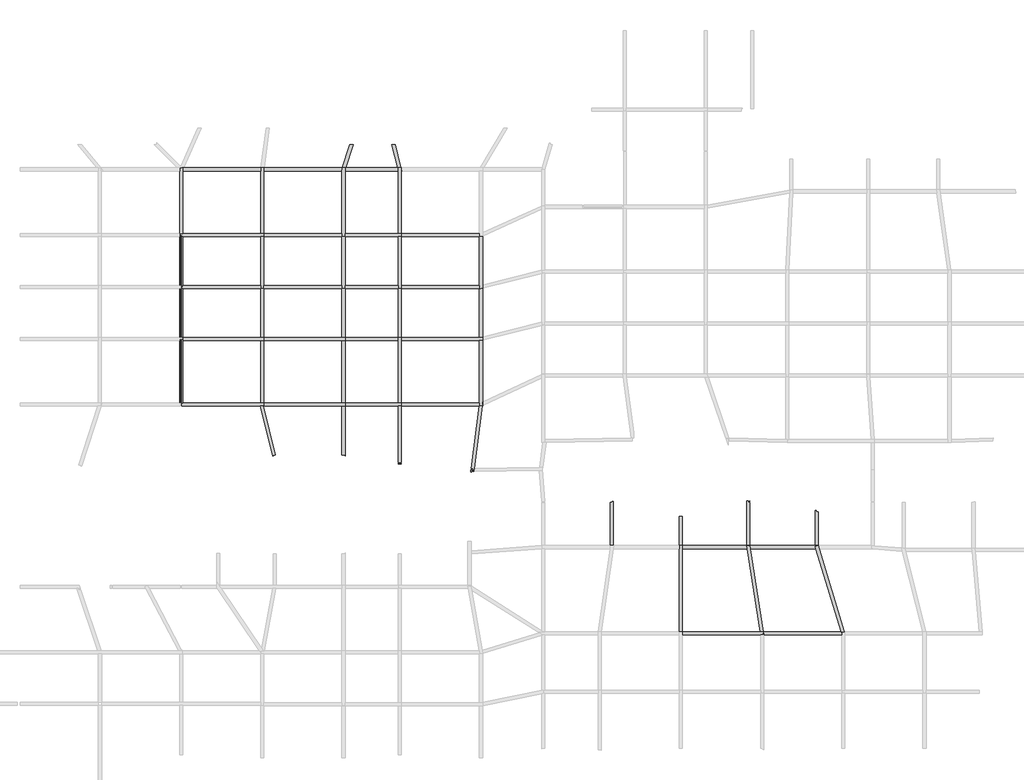
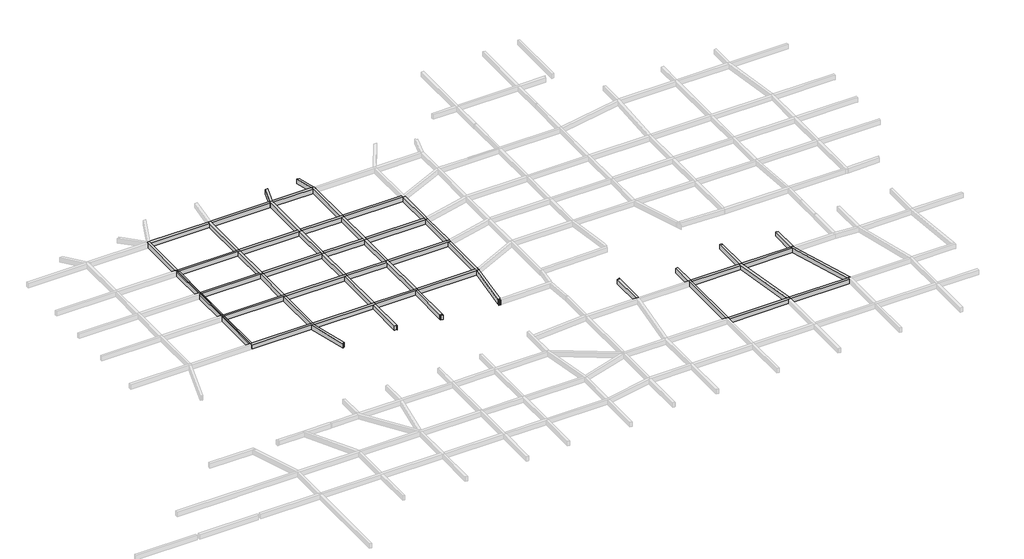
# One storey, part 11 of 15: 55 beams.
"""IFC4 building model written with IfcOpenShell, lengths in millimetres."""

from ifc_helpers import new_model, si_unit, frame, origin, place, context, project, spatial, polyline, outline, extrude, faceted_brep, element, save

model = new_model("IFC4")

# Units and contexts
model_context = context("Model", 3, world=origin())
ifc_project = project(units=[si_unit("LENGTHUNIT", "METRE", prefix="MILLI")], contexts=[model_context])

# Site, building, storey
site = spatial("IfcSite", under=ifc_project)
building = spatial("IfcBuilding", under=site)
storey = spatial("IfcBuildingStorey", under=building, Name="层高", Elevation=3300.0)

# Beams
placement = place(None, origin())
element("IfcBeam", 1, ObjectType="混凝土 - 矩形梁 : KL_beam", at=placement, inside=storey, context=model_context, shape_type="Brep", body=[
    faceted_brep([(192640.3009401, 110342.1448334, 3300.0), (192550.3215993, 110342.1448334, 3300.0), (192550.3215993, 110192.1448334, 3300.0), (192550.3215993, 104192.1448334, 3300.0), (192640.3009401, 104192.1448334, 3300.0), (192550.3215993, 104192.1448334, 2700.0), (192550.3215993, 110342.1448334, 2700.0), (192550.3215993, 110192.1448334, 2700.0), (192640.3009401, 104192.1448334, 2700.0), (192640.3009401, 110342.1448334, 2700.0)], [[[0, 1, 2, 3, 4]], [[5, 3, 2, 1, 6, 7]], [[3, 5, 8, 4]], [[0, 4, 8, 9]], [[8, 5, 7, 6, 9]], [[6, 1, 0, 9]]]),
    faceted_brep([(192850.3215993, 110342.1448334, 2700.0), (192850.3215993, 110342.1448334, 3300.0), (192850.3215993, 110192.1448334, 3300.0), (192850.3215993, 104192.1448334, 3300.0), (192850.3215993, 104192.1448334, 2700.0), (192850.3215993, 110192.1448334, 2700.0), (192760.3009401, 110342.1448334, 2700.0), (192760.3009401, 104192.1448334, 2700.0), (192760.3009401, 110342.1448334, 3300.0), (192760.3009401, 104192.1448334, 3300.0)], [[[0, 1, 2, 3, 4, 5]], [[6, 0, 5, 4, 7]], [[1, 0, 6, 8]], [[8, 6, 7, 9]], [[1, 8, 9, 3, 2]], [[4, 3, 9, 7]]]),
])
element("IfcBeam", 2, ObjectType="混凝土 - 矩形梁 : KL_beam", at=placement, inside=storey, context=model_context, shape_type="Brep", body=[
    faceted_brep([(192850.3009401, 110492.1448334, 3300.0), (192850.3112697, 110342.1448326, 3300.0), (192850.3215993, 110192.1448334, 3300.0), (200350.3215993, 110192.1448334, 3300.0), (200650.3215993, 110192.1448334, 3300.0), (200650.3215993, 110492.1448334, 3300.0), (200350.3009401, 110492.1448334, 3300.0), (192850.3215993, 110192.1448334, 2700.0), (200350.3215993, 110192.1448334, 2700.0), (200650.3215993, 110192.1448334, 2700.0), (192850.3112697, 110342.1448326, 2700.0), (192850.3009401, 110492.1448334, 2700.0), (200350.3009401, 110492.1448334, 2700.0), (200650.3215993, 110492.1448334, 2700.0)], [[[0, 1, 2, 3, 4, 5, 6]], [[2, 7, 8, 9, 4, 3]], [[7, 10, 11, 12, 13, 9, 8]], [[5, 13, 12, 11, 0, 6]], [[0, 11, 10, 7, 2, 1]], [[5, 4, 9, 13]]]),
])
element("IfcBeam", 3, ObjectType="混凝土 - 矩形梁 : KL_beam", at=placement, inside=storey, context=model_context, shape_type="Brep", body=[
    faceted_brep([(200650.3215993, 103892.1448334, 3300.0), (200650.3215993, 104192.1448334, 3300.0), (200350.3215993, 104192.1448334, 3300.0), (192850.3215993, 104192.1448334, 3300.0), (192760.3009401, 104192.1448334, 3300.0), (192760.3009401, 103892.1448334, 3300.0), (200283.1287554, 103892.1448334, 3300.0), (200592.3128442, 103892.1448334, 3300.0), (200650.3215993, 103892.1448334, 2700.0), (192760.3009401, 103892.1448334, 2700.0), (200283.1287554, 103892.1448334, 2700.0), (200592.3128442, 103892.1448334, 2700.0), (200650.3215993, 104192.1448334, 2700.0), (192760.3009401, 104192.1448334, 2700.0), (192850.3215993, 104192.1448334, 2700.0), (200350.3215993, 104192.1448334, 2700.0)], [[[0, 1, 2, 3, 4, 5, 6, 7]], [[8, 0, 7, 6, 5, 9, 10, 11]], [[12, 8, 11, 10, 9, 13, 14, 15]], [[1, 12, 15, 14, 13, 4, 3, 2]], [[1, 0, 8, 12]], [[5, 4, 13, 9]]]),
])
element("IfcBeam", 4, ObjectType="混凝土 - 矩形梁 : KL_beam", at=placement, inside=storey, context=model_context, shape_type="SweptSolid", body=[
    extrude(outline(polyline([(200350.3215993, 110192.1448334), (200650.3215993, 110192.1448334), (200650.3215993, 104192.1448334), (200350.3215993, 104192.1448334), (200350.3215993, 110192.1448334)])), frame((0.0, 0.0, 2700.0), z_axis=(0.0, 0.0, 1.0), x_axis=(1.0, 0.0, 0.0)), (0.0, 0.0, 1.0), 600.0),
])
element("IfcBeam", 5, ObjectType="混凝土 - 矩形梁 : KL_beam", at=placement, inside=storey, context=model_context, shape_type="Brep", body=[
    faceted_brep([(208450.3009398, 103892.1448334, 3300.0), (208450.3009398, 104192.1448334, 3300.0), (208150.3009398, 104192.1448334, 3300.0), (200650.3215993, 104192.1448334, 3300.0), (200650.3215993, 103892.1448334, 3300.0), (208150.3009398, 103892.1448334, 3300.0), (208450.3009398, 103892.1448334, 2700.0), (200650.3215993, 103892.1448334, 2700.0), (208150.3009398, 103892.1448334, 2700.0), (208450.3009398, 104192.1448334, 2700.0), (200650.3215993, 104192.1448334, 2700.0), (208150.3009398, 104192.1448334, 2700.0)], [[[0, 1, 2, 3, 4, 5]], [[6, 0, 5, 4, 7, 8]], [[9, 6, 8, 7, 10, 11]], [[1, 9, 11, 10, 3, 2]], [[4, 3, 10, 7]], [[1, 0, 6, 9]]]),
])
element("IfcBeam", 6, ObjectType="混凝土 - 矩形梁 : KL_beam", at=placement, inside=storey, context=model_context, shape_type="Brep", body=[
    faceted_brep([(208450.3009398, 110192.1448334, 3300.0), (208450.3009398, 110492.1448334, 3300.0), (208150.3009398, 110492.1448334, 3300.0), (200650.3215993, 110492.1448334, 3300.0), (200650.3215993, 110192.1448334, 3300.0), (208150.3009398, 110192.1448334, 3300.0), (208450.3009398, 110192.1448334, 2700.0), (200650.3215993, 110192.1448334, 2700.0), (208150.3009398, 110192.1448334, 2700.0), (208450.3009398, 110492.1448334, 2700.0), (200650.3215993, 110492.1448334, 2700.0), (208150.3009398, 110492.1448334, 2700.0)], [[[0, 1, 2, 3, 4, 5]], [[6, 0, 5, 4, 7, 8]], [[9, 6, 8, 7, 10, 11]], [[1, 9, 11, 10, 3, 2]], [[4, 3, 10, 7]], [[1, 0, 6, 9]]]),
])
element("IfcBeam", 7, ObjectType="混凝土 - 矩形梁 : KL_beam", at=placement, inside=storey, context=model_context, shape_type="SweptSolid", body=[
    extrude(outline(polyline([(208450.3009398, 104192.1448334), (208150.3009398, 104192.1448334), (208150.3009398, 110192.1448334), (208450.3009398, 110192.1448334), (208450.3009398, 104192.1448334)])), frame((0.0, 0.0, 2700.0), z_axis=(0.0, 0.0, 1.0), x_axis=(1.0, 0.0, 0.0)), (0.0, 0.0, 1.0), 600.0),
])
element("IfcBeam", 8, ObjectType="混凝土 - 矩形梁 : KL_beam", at=placement, inside=storey, context=model_context, shape_type="Brep", body=[
    faceted_brep([(213850.3009384, 103892.1448334, 3300.0), (213850.3009384, 104192.1448334, 3300.0), (213550.3009384, 104192.1448334, 3300.0), (208450.3009398, 104192.1448334, 3300.0), (208450.3009398, 103892.1448334, 3300.0), (213550.3009384, 103892.1448334, 3300.0), (213850.3009384, 103892.1448334, 2700.0), (208450.3009398, 103892.1448334, 2700.0), (213550.3009384, 103892.1448334, 2700.0), (213850.3009384, 104192.1448334, 2700.0), (208450.3009398, 104192.1448334, 2700.0), (213550.3009384, 104192.1448334, 2700.0)], [[[0, 1, 2, 3, 4, 5]], [[6, 0, 5, 4, 7, 8]], [[9, 6, 8, 7, 10, 11]], [[1, 9, 11, 10, 3, 2]], [[4, 3, 10, 7]], [[1, 0, 6, 9]]]),
])
element("IfcBeam", 9, ObjectType="混凝土 - 矩形梁 : KL_beam", at=placement, inside=storey, context=model_context, shape_type="Brep", body=[
    faceted_brep([(213850.3009384, 110492.1448334, 3300.0), (213550.3009384, 110492.1448334, 3300.0), (213550.3009384, 110192.1448334, 3300.0), (213550.3009384, 104192.1448334, 3300.0), (213850.3009384, 104192.1448334, 3300.0), (213850.3009384, 110192.1448334, 3300.0), (213850.3009384, 110492.1448334, 2700.0), (213850.3009384, 104192.1448334, 2700.0), (213850.3009384, 110192.1448334, 2700.0), (213550.3009384, 110492.1448334, 2700.0), (213550.3009384, 104192.1448334, 2700.0), (213550.3009384, 110192.1448334, 2700.0)], [[[0, 1, 2, 3, 4, 5]], [[6, 0, 5, 4, 7, 8]], [[9, 6, 8, 7, 10, 11]], [[1, 9, 11, 10, 3, 2]], [[4, 3, 10, 7]], [[1, 0, 6, 9]]]),
])
element("IfcBeam", 10, ObjectType="混凝土 - 矩形梁 : KL_beam", at=placement, inside=storey, context=model_context, shape_type="SweptSolid", body=[
    extrude(outline(polyline([(208450.3009398, 110192.1448334), (208450.3009398, 110492.1448334), (213550.3009384, 110492.1448334), (213550.3009384, 110192.1448334), (208450.3009398, 110192.1448334)])), frame((0.0, 0.0, 2700.0), z_axis=(0.0, 0.0, 1.0), x_axis=(1.0, 0.0, 0.0)), (0.0, 0.0, 1.0), 600.0),
])
element("IfcBeam", 11, ObjectType="混凝土 - 矩形梁 : KL_beam", at=placement, inside=storey, context=model_context, shape_type="SweptSolid", body=[
    extrude(outline(polyline([(213850.3009384, 98342.0955388), (213550.3009384, 98342.0955388), (213550.3009384, 98382.0955388), (213850.3009384, 98382.0955388), (213850.3009384, 98342.0955388)])), frame((0.0, 0.0, 2700.0), z_axis=(0.0, 0.0, 1.0), x_axis=(1.0, 0.0, 0.0)), (0.0, 0.0, 1.0), 600.0),
    extrude(outline(polyline([(213550.3009384, 103892.1448334), (213850.3009384, 103892.1448334), (213850.3009384, 98502.0955388), (213550.3009384, 98502.0955388), (213550.3009384, 103892.1448334)])), frame((0.0, 0.0, 2700.0), z_axis=(0.0, 0.0, 1.0), x_axis=(1.0, 0.0, 0.0)), (0.0, 0.0, 1.0), 600.0),
])
element("IfcBeam", 12, ObjectType="混凝土 - 矩形梁 : KL_beam", at=placement, inside=storey, context=model_context, shape_type="Brep", body=[
    faceted_brep([(208450.3009398, 103892.1448334, 3300.0), (208150.3009398, 103892.1448334, 3300.0), (208150.3009398, 99202.0955388, 3300.0), (208329.2467743, 99202.0955388, 3300.0), (208449.2467743, 99202.0955388, 3300.0), (208449.2467743, 99082.0955388, 3300.0), (208450.3009398, 99082.0955388, 3300.0), (208150.3009398, 103892.1448334, 2700.0), (208150.3009398, 99202.0955388, 2700.0), (208450.3009398, 103892.1448334, 2700.0), (208450.3009398, 99082.0955388, 2700.0), (208449.2467743, 99082.0955388, 2700.0), (208449.2467743, 99202.0955388, 2700.0)], [[[0, 1, 2, 3, 4, 5, 6]], [[1, 7, 8, 2]], [[7, 9, 10, 11, 12, 8]], [[9, 0, 6, 10]], [[1, 0, 9, 7]], [[10, 6, 5, 11]], [[2, 8, 12, 4, 3]], [[4, 12, 11, 5]]]),
])
element("IfcBeam", 13, ObjectType="混凝土 - 矩形梁 : KL_beam", at=placement, inside=storey, context=model_context, shape_type="SweptSolid", body=[
    extrude(outline(polyline([(200283.1287554, 103892.1448334), (200592.3128442, 103892.1448334), (201761.673468, 99202.0955388), (201562.0411038, 99202.0955388), (201562.0411038, 99082.0955388), (201482.4087396, 99082.0955388), (200283.1287554, 103892.1448334)])), frame((0.0, 0.0, 2700.0), z_axis=(0.0, 0.0, 1.0), x_axis=(1.0, 0.0, 0.0)), (0.0, 0.0, 1.0), 600.0),
])
element("IfcBeam", 14, ObjectType="混凝土 - 矩形梁 : KL_beam", at=placement, inside=storey, context=model_context, shape_type="Brep", body=[
    faceted_brep([(200650.3009401, 120192.1448334, 3300.0), (200650.3009401, 120492.1448334, 3300.0), (200350.3009384, 120492.1448334, 3300.0), (192850.3052169, 120492.1448334, 3300.0), (192550.3009401, 120492.1448334, 3300.0), (192550.3009401, 120192.1448334, 3300.0), (192640.3009401, 120192.1448334, 3300.0), (192640.3009401, 120342.1448334, 3300.0), (192760.3009401, 120342.1448334, 3300.0), (192760.3009401, 120192.1448334, 3300.0), (192850.3009401, 120192.1448334, 3300.0), (200350.3009401, 120192.1448334, 3300.0), (200650.3009401, 120192.1448334, 2700.0), (192760.3009401, 120192.1448334, 2700.0), (192850.3009401, 120192.1448334, 2700.0), (200350.3009401, 120192.1448334, 2700.0), (200650.3009401, 120492.1448334, 2700.0), (192760.3009401, 120342.1448334, 2700.0), (192640.3009401, 120342.1448334, 2700.0), (192640.3009401, 120192.1448334, 2700.0), (192550.3009401, 120192.1448334, 2700.0), (192550.3009401, 120492.1448334, 2700.0), (192850.3052169, 120492.1448334, 2700.0), (200350.3009384, 120492.1448334, 2700.0)], [[[0, 1, 2, 3, 4, 5, 6, 7, 8, 9, 10, 11]], [[12, 0, 11, 10, 9, 13, 14, 15]], [[16, 12, 15, 14, 13, 17, 18, 19, 20, 21, 22, 23]], [[1, 16, 23, 22, 21, 4, 3, 2]], [[1, 0, 12, 16]], [[5, 4, 21, 20]], [[18, 7, 6, 19]], [[8, 17, 13, 9]], [[7, 18, 17, 8]], [[5, 20, 19, 6]]]),
])
element("IfcBeam", 15, ObjectType="混凝土 - 矩形梁 : KL_beam", at=placement, inside=storey, context=model_context, shape_type="Brep", body=[
    faceted_brep([(200350.3009401, 115192.1448334, 3300.0), (200650.3009401, 115192.1448334, 3300.0), (200650.3009401, 115492.1448334, 3300.0), (200650.3009401, 120192.1448334, 3300.0), (200350.3009401, 120192.1448334, 3300.0), (200350.3009401, 115492.1448334, 3300.0), (200350.3009401, 115192.1448334, 2700.0), (200350.3009401, 120192.1448334, 2700.0), (200350.3009401, 115492.1448334, 2700.0), (200650.3009401, 115192.1448334, 2700.0), (200650.3009401, 120192.1448334, 2700.0), (200650.3009401, 115492.1448334, 2700.0)], [[[0, 1, 2, 3, 4, 5]], [[6, 0, 5, 4, 7, 8]], [[9, 6, 8, 7, 10, 11]], [[1, 9, 11, 10, 3, 2]], [[4, 3, 10, 7]], [[1, 0, 6, 9]]]),
])
element("IfcBeam", 16, ObjectType="混凝土 - 矩形梁 : KL_beam", at=placement, inside=storey, context=model_context, shape_type="Brep", body=[
    faceted_brep([(200650.3009384, 126792.1448334, 3300.0), (200368.9005343, 126792.1448334, 3300.0), (200350.3009384, 126792.1448334, 3300.0), (200350.3009384, 126492.1448334, 3300.0), (200350.3009384, 120492.1448334, 3300.0), (200650.3009384, 120492.1448334, 3300.0), (200650.3009384, 126492.1448334, 3300.0), (200350.3009384, 126792.1448334, 2700.0), (200350.3009384, 126492.1448334, 2700.0), (200350.3009384, 120492.1448334, 2700.0), (200368.9005343, 126792.1448334, 2700.0), (200650.3009384, 126792.1448334, 2700.0), (200650.3009384, 126492.1448334, 2700.0), (200650.3009384, 120492.1448334, 2700.0)], [[[0, 1, 2, 3, 4, 5, 6]], [[2, 7, 8, 9, 4, 3]], [[7, 10, 11, 12, 13, 9, 8]], [[11, 0, 6, 5, 13, 12]], [[5, 4, 9, 13]], [[2, 1, 0, 11, 10, 7]]]),
])
element("IfcBeam", 17, ObjectType="混凝土 - 矩形梁 : KL_beam", at=placement, inside=storey, context=model_context, shape_type="Brep", body=[
    faceted_brep([(192850.3052169, 126792.1448334, 3300.0), (192762.4372513, 126792.1448334, 3300.0), (192550.3052169, 126792.1448334, 3300.0), (192550.3052169, 126492.1448334, 3300.0), (192550.3052169, 120492.1448334, 3300.0), (192850.3052169, 120492.1448334, 3300.0), (192850.3052169, 126492.1448334, 3300.0), (192550.3052169, 126792.1448334, 2700.0), (192550.3052169, 126492.1448334, 2700.0), (192550.3052169, 120492.1448334, 2700.0), (192762.4372513, 126792.1448334, 2700.0), (192850.3052169, 126792.1448334, 2700.0), (192850.3052169, 126492.1448334, 2700.0), (192850.3052169, 120492.1448334, 2700.0)], [[[0, 1, 2, 3, 4, 5, 6]], [[2, 7, 8, 9, 4, 3]], [[7, 10, 11, 12, 13, 9, 8]], [[11, 0, 6, 5, 13, 12]], [[5, 4, 9, 13]], [[2, 1, 0, 11, 10, 7]]]),
])
element("IfcBeam", 18, ObjectType="混凝土 - 矩形梁 : KL_beam", at=placement, inside=storey, context=model_context, shape_type="Brep", body=[
    faceted_brep([(200350.3009384, 126492.1448334, 3300.0), (200350.3009384, 126792.1448334, 3300.0), (192931.5266601, 126792.1448334, 3300.0), (192850.3052169, 126792.1448334, 3300.0), (192850.3052169, 126492.1448334, 3300.0), (200350.3009384, 126492.1448334, 2700.0), (192850.3052169, 126492.1448334, 2700.0), (200350.3009384, 126792.1448334, 2700.0), (192850.3052169, 126792.1448334, 2700.0), (192931.5266601, 126792.1448334, 2700.0)], [[[0, 1, 2, 3, 4]], [[5, 0, 4, 6]], [[7, 5, 6, 8, 9]], [[1, 7, 9, 8, 3, 2]], [[1, 0, 5, 7]], [[4, 3, 8, 6]]]),
])
element("IfcBeam", 19, ObjectType="混凝土 - 矩形梁 : KL_beam", at=placement, inside=storey, context=model_context, shape_type="Brep", body=[
    faceted_brep([(208150.3009398, 120192.1448334, 3300.0), (208450.3009398, 120192.1448334, 3300.0), (208450.3009398, 120492.1448334, 3300.0), (208450.3009398, 126492.1448334, 3300.0), (208450.3009398, 126792.1448334, 3300.0), (208191.3195606, 126792.1448334, 3300.0), (208150.3009398, 126792.1448334, 3300.0), (208150.3009398, 126665.9024994, 3300.0), (208150.3009398, 126492.1448334, 3300.0), (208150.3009398, 120492.1448334, 3300.0), (208150.3009398, 120192.1448334, 2700.0), (208150.3009398, 126792.1448334, 2700.0), (208150.3009398, 126665.9024994, 2700.0), (208150.3009398, 126492.1448334, 2700.0), (208150.3009398, 120492.1448334, 2700.0), (208450.3009398, 120192.1448334, 2700.0), (208191.3195606, 126792.1448334, 2700.0), (208450.3009398, 126792.1448334, 2700.0), (208450.3009398, 126492.1448334, 2700.0), (208450.3009398, 120492.1448334, 2700.0)], [[[0, 1, 2, 3, 4, 5, 6, 7, 8, 9]], [[10, 0, 9, 8, 7, 6, 11, 12, 13, 14]], [[15, 10, 14, 13, 12, 11, 16, 17, 18, 19]], [[1, 15, 19, 18, 17, 4, 3, 2]], [[1, 0, 10, 15]], [[6, 5, 4, 17, 16, 11]]]),
])
element("IfcBeam", 20, ObjectType="混凝土 - 矩形梁 : KL_beam", at=placement, inside=storey, context=model_context, shape_type="Brep", body=[
    faceted_brep([(213850.3009384, 120192.1448334, 3300.0), (213850.3009384, 120492.1448334, 3300.0), (213550.3009384, 120492.1448334, 3300.0), (208450.3009398, 120492.1448334, 3300.0), (208450.3009398, 120192.1448334, 3300.0), (213550.3009384, 120192.1448334, 3300.0), (213850.3009384, 120192.1448334, 2700.0), (208450.3009398, 120192.1448334, 2700.0), (213550.3009384, 120192.1448334, 2700.0), (213850.3009384, 120492.1448334, 2700.0), (208450.3009398, 120492.1448334, 2700.0), (213550.3009384, 120492.1448334, 2700.0)], [[[0, 1, 2, 3, 4, 5]], [[6, 0, 5, 4, 7, 8]], [[9, 6, 8, 7, 10, 11]], [[1, 9, 11, 10, 3, 2]], [[4, 3, 10, 7]], [[1, 0, 6, 9]]]),
])
element("IfcBeam", 21, ObjectType="混凝土 - 矩形梁 : KL_beam", at=placement, inside=storey, context=model_context, shape_type="Brep", body=[
    faceted_brep([(213850.3009384, 126792.1448334, 3300.0), (213817.4937825, 126792.1448334, 3300.0), (213550.3009384, 126792.1448334, 3300.0), (213550.3009384, 126492.1448334, 3300.0), (213550.3009384, 120492.1448334, 3300.0), (213850.3009384, 120492.1448334, 3300.0), (213850.3009384, 126492.1448336, 3300.0), (213850.3009384, 126660.5625177, 3300.0), (213550.3009384, 126792.1448334, 2700.0), (213550.3009384, 126492.1448334, 2700.0), (213550.3009384, 120492.1448334, 2700.0), (213817.4937825, 126792.1448334, 2700.0), (213850.3009384, 126792.1448334, 2700.0), (213850.3009384, 126660.5625177, 2700.0), (213850.3009384, 126492.1448336, 2700.0), (213850.3009384, 120492.1448334, 2700.0)], [[[0, 1, 2, 3, 4, 5, 6, 7]], [[2, 8, 9, 10, 4, 3]], [[8, 11, 12, 13, 14, 15, 10, 9]], [[12, 0, 7, 6, 5, 15, 14, 13]], [[5, 4, 10, 15]], [[2, 1, 0, 12, 11, 8]]]),
])
element("IfcBeam", 22, ObjectType="混凝土 - 矩形梁 : KL_beam", at=placement, inside=storey, context=model_context, shape_type="Brep", body=[
    faceted_brep([(208450.3009398, 126792.1448334, 3300.0), (208450.3009398, 126492.1448334, 3300.0), (213550.3009384, 126492.1448334, 3300.0), (213550.3009384, 126792.1448334, 3300.0), (213508.3096937, 126792.1448334, 3300.0), (208506.7582279, 126792.1448334, 3300.0), (208450.3009398, 126492.1448334, 2700.0), (213550.3009384, 126492.1448334, 2700.0), (208450.3009398, 126792.1448334, 2700.0), (208506.7582279, 126792.1448334, 2700.0), (213508.3096937, 126792.1448334, 2700.0), (213550.3009384, 126792.1448334, 2700.0)], [[[0, 1, 2, 3, 4, 5]], [[1, 6, 7, 2]], [[6, 8, 9, 10, 11, 7]], [[8, 0, 5, 4, 3, 11, 10, 9]], [[1, 0, 8, 6]], [[3, 2, 7, 11]]]),
])
element("IfcBeam", 23, ObjectType="混凝土 - 矩形梁 : KL_beam", at=placement, inside=storey, context=model_context, shape_type="Brep", body=[
    faceted_brep([(209233.0793093, 129027.5312684, 3300.0), (208917.640642, 129027.5312684, 3300.0), (208191.3195606, 126792.1448334, 3300.0), (208450.3009398, 126792.1448334, 3300.0), (208506.7582279, 126792.1448334, 3300.0), (209233.0793093, 129027.5312684, 2700.0), (208506.7582279, 126792.1448334, 2700.0), (208917.640642, 129027.5312684, 2700.0), (208450.3009398, 126792.1448334, 2700.0), (208191.3195606, 126792.1448334, 2700.0)], [[[0, 1, 2, 3, 4]], [[5, 0, 4, 6]], [[7, 5, 6, 8, 9]], [[1, 7, 9, 2]], [[1, 0, 5, 7]], [[2, 9, 8, 6, 4, 3]]]),
    faceted_brep([(208150.3009398, 126492.1448334, 2700.0), (208150.3009398, 126492.1448334, 3300.0), (208093.8436517, 126492.1448334, 3300.0), (208093.8436517, 126492.1448334, 2700.0), (208150.3009398, 126665.9024994, 3300.0), (208150.3009398, 126665.9024994, 2700.0)], [[[0, 1, 2, 3]], [[4, 1, 0, 5]], [[4, 2, 1]], [[3, 5, 0]], [[2, 4, 5, 3]]]),
])
element("IfcBeam", 24, ObjectType="混凝土 - 矩形梁 : KL_beam", at=placement, inside=storey, context=model_context, shape_type="Brep", body=[
    faceted_brep([(213260.149347, 129027.5312684, 3300.0), (212950.9652582, 129027.5312684, 3300.0), (213508.3096937, 126792.1448334, 3300.0), (213550.3009384, 126792.1448334, 3300.0), (213817.4937825, 126792.1448334, 3300.0), (213817.4937825, 126792.1448334, 2700.0), (213260.149347, 129027.5312684, 2700.0), (212950.9652582, 129027.5312684, 2700.0), (213550.3009384, 126792.1448334, 2700.0), (213508.3096937, 126792.1448334, 2700.0)], [[[0, 1, 2, 3, 4]], [[4, 5, 6, 0]], [[7, 6, 5, 8, 9]], [[1, 7, 9, 2]], [[0, 6, 7, 1]], [[5, 4, 3, 2, 9, 8]]]),
    faceted_brep([(213850.3009384, 126492.1448336, 3300.0), (213850.3009384, 126660.5625177, 3300.0), (213850.3009384, 126660.5625177, 2700.0), (213850.3009384, 126492.1448336, 2700.0), (213892.2921833, 126492.1448336, 2700.0), (213892.2921833, 126492.1448336, 3300.0)], [[[0, 1, 2, 3]], [[4, 5, 0, 3]], [[5, 1, 0]], [[1, 5, 4, 2]], [[2, 4, 3]]]),
])
element("IfcBeam", 25, ObjectType="混凝土 - 矩形梁 : KL_beam", at=placement, inside=storey, context=model_context, shape_type="SweptSolid", body=[
    extrude(outline(polyline([(213850.3009384, 120192.1448334), (213850.3009384, 120492.1448334), (221350.3009384, 120492.1448334), (221350.3009384, 120192.1448334), (213850.3009384, 120192.1448334)])), frame((0.0, 0.0, 2700.0), z_axis=(0.0, 0.0, 1.0), x_axis=(1.0, 0.0, 0.0)), (0.0, 0.0, 1.0), 600.0),
])
element("IfcBeam", 26, ObjectType="混凝土 - 矩形梁 : KL_beam", at=placement, inside=storey, context=model_context, shape_type="Brep", body=[
    faceted_brep([(221350.3009384, 115192.1448334, 3300.0), (221518.7623395, 115192.1448334, 3300.0), (221650.3009384, 115192.1448334, 3300.0), (221650.3009384, 115225.0213279, 3300.0), (221650.3009384, 115534.2497393, 3300.0), (221650.3009384, 120192.1448334, 3300.0), (221350.3009384, 120192.1448334, 3300.0), (221350.3009384, 115492.1448334, 3300.0), (221650.3009384, 115192.1448334, 2700.0), (221650.3009384, 115225.0213279, 2700.0), (221650.3009384, 115534.2497393, 2700.0), (221650.3009384, 120192.1448334, 2700.0), (221518.7623395, 115192.1448334, 2700.0), (221350.3009384, 115192.1448334, 2700.0), (221350.3009384, 115492.1448334, 2700.0), (221350.3009384, 120192.1448334, 2700.0)], [[[0, 1, 2, 3, 4, 5, 6, 7]], [[2, 8, 9, 10, 11, 5, 4, 3]], [[8, 12, 13, 14, 15, 11, 10, 9]], [[13, 0, 7, 6, 15, 14]], [[6, 5, 11, 15]], [[2, 1, 0, 13, 12, 8]]]),
])
element("IfcBeam", 27, ObjectType="混凝土 - 矩形梁 : KL_beam", at=placement, inside=storey, context=model_context, shape_type="Brep", body=[
    faceted_brep([(213550.3009384, 115192.1448334, 3300.0), (213850.3009384, 115192.1448334, 3300.0), (213850.3009384, 115492.1448334, 3300.0), (213850.3009384, 120192.1448334, 3300.0), (213550.3009384, 120192.1448334, 3300.0), (213550.3009384, 115492.1448334, 3300.0), (213550.3009384, 115192.1448334, 2700.0), (213550.3009384, 120192.1448334, 2700.0), (213550.3009384, 115492.1448334, 2700.0), (213850.3009384, 115192.1448334, 2700.0), (213850.3009384, 120192.1448334, 2700.0), (213850.3009384, 115492.1448334, 2700.0)], [[[0, 1, 2, 3, 4, 5]], [[6, 0, 5, 4, 7, 8]], [[9, 6, 8, 7, 10, 11]], [[1, 9, 11, 10, 3, 2]], [[4, 3, 10, 7]], [[1, 0, 6, 9]]]),
])
element("IfcBeam", 28, ObjectType="混凝土 - 矩形梁 : KL_beam", at=placement, inside=storey, context=model_context, shape_type="SweptSolid", body=[
    extrude(outline(polyline([(221350.3009384, 115492.1448334), (221350.3009384, 115192.1448334), (213850.3009384, 115192.1448334), (213850.3009384, 115492.1448334), (221350.3009384, 115492.1448334)])), frame((0.0, 0.0, 2700.0), z_axis=(0.0, 0.0, 1.0), x_axis=(1.0, 0.0, 0.0)), (0.0, 0.0, 1.0), 600.0),
])
element("IfcBeam", 29, ObjectType="混凝土 - 矩形梁 : KL_beam", at=placement, inside=storey, context=model_context, shape_type="Brep", body=[
    faceted_brep([(208150.3009398, 115192.1448334, 3300.0), (208450.3009398, 115192.1448334, 3300.0), (208450.3009398, 115492.1448334, 3300.0), (208450.3009398, 120192.1448334, 3300.0), (208150.3009398, 120192.1448334, 3300.0), (208150.3009398, 115492.1448334, 3300.0), (208450.3009398, 115192.1448334, 2700.0), (208450.3009398, 115492.1448334, 2700.0), (208450.3009398, 120192.1448334, 2700.0), (208150.3009398, 115192.1448334, 2700.0), (208150.3009398, 115492.1448334, 2700.0), (208150.3009398, 120192.1448334, 2700.0)], [[[0, 1, 2, 3, 4, 5]], [[1, 6, 7, 8, 3, 2]], [[6, 9, 10, 11, 8, 7]], [[9, 0, 5, 4, 11, 10]], [[4, 3, 8, 11]], [[1, 0, 9, 6]]]),
])
element("IfcBeam", 30, ObjectType="混凝土 - 矩形梁 : KL_beam", at=placement, inside=storey, context=model_context, shape_type="SweptSolid", body=[
    extrude(outline(polyline([(213550.3009384, 115492.1448334), (213550.3009384, 115192.1448334), (208450.3009398, 115192.1448334), (208450.3009398, 115492.1448334), (213550.3009384, 115492.1448334)])), frame((0.0, 0.0, 2700.0), z_axis=(0.0, 0.0, 1.0), x_axis=(1.0, 0.0, 0.0)), (0.0, 0.0, 1.0), 600.0),
])
element("IfcBeam", 31, ObjectType="混凝土 - 矩形梁 : KL_beam", at=placement, inside=storey, context=model_context, shape_type="SweptSolid", body=[
    extrude(outline(polyline([(200650.3009401, 120192.1448334), (200650.3009401, 120492.1448334), (208150.3009398, 120492.1448334), (208150.3009398, 120192.1448334), (200650.3009401, 120192.1448334)])), frame((0.0, 0.0, 2700.0), z_axis=(0.0, 0.0, 1.0), x_axis=(1.0, 0.0, 0.0)), (0.0, 0.0, 1.0), 600.0),
])
element("IfcBeam", 32, ObjectType="混凝土 - 矩形梁 : KL_beam", at=placement, inside=storey, context=model_context, shape_type="Brep", body=[
    faceted_brep([(200650.3009384, 126492.1448334, 3300.0), (200650.3009384, 126492.1448334, 2700.0), (208093.8436517, 126492.1448334, 2700.0), (208093.8436517, 126492.1448334, 3300.0), (200650.3009384, 126792.1448334, 3300.0), (200650.3009384, 126792.1448334, 2700.0), (208150.3009398, 126792.1448334, 2700.0), (208150.3009398, 126792.1448334, 3300.0), (208150.3009398, 126665.9024994, 3300.0), (208150.3009398, 126665.9024994, 2700.0), (200671.5332885, 126792.1448334, 3300.0), (200671.5332885, 126792.1448334, 2700.0)], [[[0, 1, 2, 3]], [[0, 4, 5, 1]], [[6, 7, 8, 9]], [[4, 0, 3, 8, 7, 10]], [[1, 5, 11, 6, 9, 2]], [[5, 4, 10, 7, 6, 11]], [[3, 2, 9, 8]]]),
])
element("IfcBeam", 33, ObjectType="混凝土 - 矩形梁 : KL_beam", at=placement, inside=storey, context=model_context, shape_type="SweptSolid", body=[
    extrude(outline(polyline([(200650.3009401, 110492.1448334), (200350.3009401, 110492.1448334), (200350.3009401, 115192.1448334), (200650.3009401, 115192.1448334), (200650.3009401, 110492.1448334)])), frame((0.0, 0.0, 2700.0), z_axis=(0.0, 0.0, 1.0), x_axis=(1.0, 0.0, 0.0)), (0.0, 0.0, 1.0), 600.0),
])
element("IfcBeam", 34, ObjectType="混凝土 - 矩形梁 : KL_beam", at=placement, inside=storey, context=model_context, shape_type="SweptSolid", body=[
    extrude(outline(polyline([(208450.3009398, 110492.1448334), (208150.3009398, 110492.1448334), (208150.3009398, 115192.1448334), (208450.3009398, 115192.1448334), (208450.3009398, 110492.1448334)])), frame((0.0, 0.0, 2700.0), z_axis=(0.0, 0.0, 1.0), x_axis=(1.0, 0.0, 0.0)), (0.0, 0.0, 1.0), 600.0),
])
element("IfcBeam", 35, ObjectType="混凝土 - 矩形梁 : KL_beam", at=placement, inside=storey, context=model_context, shape_type="SweptSolid", body=[
    extrude(outline(polyline([(200650.3009401, 115192.1448334), (200650.3009401, 115492.1448334), (208150.3009398, 115492.1448334), (208150.3009398, 115192.1448334), (200650.3009401, 115192.1448334)])), frame((0.0, 0.0, 2700.0), z_axis=(0.0, 0.0, 1.0), x_axis=(1.0, 0.0, 0.0)), (0.0, 0.0, 1.0), 600.0),
])
element("IfcBeam", 36, ObjectType="混凝土 - 矩形梁 : KL_beam", at=placement, inside=storey, context=model_context, shape_type="SweptSolid", body=[
    extrude(outline(polyline([(213850.3009384, 110492.1448334), (213550.3009384, 110492.1448334), (213550.3009384, 115192.1448334), (213850.3009384, 115192.1448334), (213850.3009384, 110492.1448334)])), frame((0.0, 0.0, 2700.0), z_axis=(0.0, 0.0, 1.0), x_axis=(1.0, 0.0, 0.0)), (0.0, 0.0, 1.0), 600.0),
])
element("IfcBeam", 37, ObjectType="混凝土 - 矩形梁 : KL_beam", at=placement, inside=storey, context=model_context, shape_type="Brep", body=[
    faceted_brep([(221650.3009384, 110192.1448334, 3300.0), (221650.3009384, 110225.0213279, 3300.0), (221650.3009384, 110492.1448334, 3300.0), (221481.8395373, 110492.1448334, 3300.0), (221350.3009384, 110492.1448334, 3300.0), (213850.3009384, 110492.1448334, 3300.0), (213850.3009384, 110192.1448334, 3300.0), (221350.3009384, 110192.1448334, 3300.0), (221650.3009384, 110192.1448334, 2700.0), (213850.3009384, 110192.1448334, 2700.0), (221350.3009384, 110192.1448334, 2700.0), (221650.3009384, 110492.1448334, 2700.0), (221650.3009384, 110225.0213279, 2700.0), (213850.3009384, 110492.1448334, 2700.0), (221350.3009384, 110492.1448334, 2700.0), (221481.8395373, 110492.1448334, 2700.0)], [[[0, 1, 2, 3, 4, 5, 6, 7]], [[8, 0, 7, 6, 9, 10]], [[11, 12, 8, 10, 9, 13, 14, 15]], [[2, 11, 15, 14, 13, 5, 4, 3]], [[6, 5, 13, 9]], [[2, 1, 0, 8, 12, 11]]]),
])
element("IfcBeam", 38, ObjectType="混凝土 - 矩形梁 : KL_beam", at=placement, inside=storey, context=model_context, shape_type="Brep", body=[
    faceted_brep([(221350.3009384, 103892.1448334, 3300.0), (221632.0013714, 103892.1448334, 3300.0), (221650.3009384, 103892.1448334, 3300.0), (221650.3009384, 103946.6115658, 3300.0), (221650.3009384, 104032.4006699, 3300.0), (221650.3009384, 104277.6648839, 3300.0), (221650.3009384, 110192.1448334, 3300.0), (221350.3009384, 110192.1448334, 3300.0), (221350.3009384, 104192.1448334, 3300.0), (221650.3009384, 103892.1448334, 2700.0), (221650.3009384, 103946.6115658, 2700.0), (221650.3009384, 104032.4006699, 2700.0), (221650.3009384, 104277.6648839, 2700.0), (221650.3009384, 110192.1448334, 2700.0), (221632.0013714, 103892.1448334, 2700.0), (221350.3009384, 103892.1448334, 2700.0), (221350.3009384, 104192.1448334, 2700.0), (221350.3009384, 110192.1448334, 2700.0)], [[[0, 1, 2, 3, 4, 5, 6, 7, 8]], [[2, 9, 10, 11, 12, 13, 6, 5, 4, 3]], [[9, 14, 15, 16, 17, 13, 12, 11, 10]], [[15, 0, 8, 7, 17, 16]], [[7, 6, 13, 17]], [[2, 1, 0, 15, 14, 9]]]),
])
element("IfcBeam", 39, ObjectType="混凝土 - 矩形梁 : KL_beam", at=placement, inside=storey, context=model_context, shape_type="Brep", body=[
    faceted_brep([(213850.3009384, 104192.1448334, 3300.0), (213850.3009384, 103892.1448334, 3300.0), (221329.4586755, 103892.1448334, 3300.0), (221350.3009384, 103892.1448334, 3300.0), (221350.3009384, 104192.1448334, 3300.0), (213850.3009384, 103892.1448334, 2700.0), (221329.4586755, 103892.1448334, 2700.0), (221350.3009384, 103892.1448334, 2700.0), (213850.3009384, 104192.1448334, 2700.0), (221350.3009384, 104192.1448334, 2700.0)], [[[0, 1, 2, 3, 4]], [[1, 5, 6, 7, 3, 2]], [[5, 8, 9, 7, 6]], [[8, 0, 4, 9]], [[1, 0, 8, 5]], [[4, 3, 7, 9]]]),
])
element("IfcBeam", 40, ObjectType="混凝土 - 矩形梁 : KL_beam", at=placement, inside=storey, context=model_context, shape_type="Brep", body=[
    faceted_brep([(221684.3757671, 104293.5649694, 3300.0), (221650.3009384, 104277.6648839, 3300.0), (221650.3009384, 104192.1448334, 3300.0), (221650.3009384, 104032.4006699, 3300.0), (221650.3009384, 104032.4006699, 2700.0), (221684.3757671, 104293.5649694, 2700.0), (221650.3009384, 104277.6648839, 2700.0), (221650.3009384, 104192.1448334, 2700.0)], [[[0, 1, 2, 3]], [[3, 4, 5, 0]], [[6, 5, 4, 7]], [[4, 3, 2, 1, 6, 7]], [[0, 5, 6, 1]]]),
    faceted_brep([(221329.4586755, 103892.1448334, 3300.0), (221329.4586755, 103892.1448334, 2700.0), (220545.804913, 97885.8817439, 2700.0), (220545.804913, 97885.8817439, 3300.0), (221632.0013714, 103892.1448334, 3300.0), (221632.0013714, 103892.1448334, 2700.0), (221350.3009384, 103892.1448334, 2700.0), (221350.3009384, 103892.1448334, 3300.0), (220749.247895, 97885.8817439, 3300.0), (220749.247895, 97593.3599914, 3300.0), (220810.3205741, 97594.426019, 3300.0), (220849.5577256, 97895.1566044, 3300.0), (220810.3205741, 97594.426019, 2700.0), (220849.5577256, 97895.1566044, 2700.0), (220749.247895, 97593.3599914, 2700.0), (220749.247895, 97885.8817439, 2700.0)], [[[0, 1, 2, 3]], [[4, 5, 6, 1, 0, 7]], [[4, 7, 0, 3, 8, 9, 10, 11]], [[5, 4, 11, 10, 12, 13]], [[1, 6, 5, 13, 12, 14, 15, 2]], [[8, 15, 14, 9]], [[15, 8, 3, 2]], [[12, 10, 9, 14]]]),
    faceted_brep([(220629.247895, 97591.2653836, 3300.0), (220629.247895, 97591.2653836, 2700.0), (220629.247895, 97765.8817439, 2700.0), (220629.247895, 97765.8817439, 3300.0), (220530.148181, 97765.8817439, 2700.0), (220530.148181, 97765.8817439, 3300.0), (220507.0872915, 97589.1330623, 3300.0), (220507.0872915, 97589.1330623, 2700.0)], [[[0, 1, 2, 3]], [[4, 5, 3, 2]], [[6, 7, 1, 0]], [[7, 6, 5, 4]], [[6, 0, 3, 5]], [[1, 7, 4, 2]]]),
])
element("IfcBeam", 41, ObjectType="混凝土 - 矩形梁 : KL_beam", at=placement, inside=storey, context=model_context, shape_type="SweptSolid", body=[
    extrude(outline(polyline([(221518.7623395, 115192.1448334), (221650.3009384, 115192.1448334), (221650.3009384, 110534.2497393), (221481.8395373, 110492.1448334), (221350.3009384, 110492.1448334), (221350.3009384, 115150.0399275), (221518.7623395, 115192.1448334)])), frame((0.0, 0.0, 2700.0), z_axis=(0.0, 0.0, 1.0), x_axis=(1.0, 0.0, 0.0)), (0.0, 0.0, 1.0), 600.0),
])
element("IfcBeam", 42, ObjectType="混凝土 - 矩形梁 : KL_beam", at=placement, inside=storey, context=model_context, shape_type="Brep", body=[
    faceted_brep([(253586.3730636, 90404.1938247, 3300.0), (253651.2761679, 90191.9053361, 3300.0), (256095.4232782, 82197.4603606, 3300.0), (256149.8021771, 82019.5949965, 3300.0), (256149.8021771, 82192.0126467, 3300.0), (256410.7963384, 82192.0126467, 3300.0), (253964.9836949, 90191.9053361, 3300.0), (253873.2644904, 90491.9053361, 3300.0), (256410.7963384, 82192.0126467, 2700.0), (253964.9836949, 90191.9053361, 2700.0), (253873.2644904, 90491.9053361, 2700.0), (256149.8021771, 82019.5949965, 2700.0), (256095.4232782, 82197.4603606, 2700.0), (253651.2761679, 90191.9053361, 2700.0), (253586.3730636, 90404.1938247, 2700.0), (256149.8021771, 82192.0126467, 2700.0)], [[[0, 1, 2, 3, 4, 5, 6, 7]], [[5, 8, 9, 10, 7, 6]], [[11, 12, 13, 14, 10, 9, 8, 15]], [[3, 2, 1, 0, 14, 13, 12, 11]], [[15, 4, 3, 11]], [[4, 15, 8, 5]], [[0, 7, 10, 14]]]),
])
element("IfcBeam", 43, ObjectType="混凝土 - 矩形梁 : KL_beam", at=placement, inside=storey, context=model_context, shape_type="Brep", body=[
    faceted_brep([(200350.3009401, 115192.1448334, 3300.0), (200350.3009401, 115492.1448334, 3300.0), (192850.3009401, 115492.1448334, 3300.0), (192850.3009401, 115342.1448334, 3300.0), (192760.3009401, 115342.1448334, 3300.0), (192760.3009401, 115192.1448334, 3300.0), (192850.3009401, 115192.1448334, 3300.0), (200350.3009401, 115192.1448334, 2700.0), (192760.3009401, 115192.1448334, 2700.0), (192850.3009401, 115192.1448334, 2700.0), (200350.3009401, 115492.1448334, 2700.0), (192760.3009401, 115342.1448334, 2700.0), (192850.3009401, 115342.1448334, 2700.0), (192850.3009401, 115492.1448334, 2700.0)], [[[0, 1, 2, 3, 4, 5, 6]], [[7, 0, 6, 5, 8, 9]], [[10, 7, 9, 8, 11, 12, 13]], [[1, 10, 13, 2]], [[1, 0, 7, 10]], [[12, 3, 2, 13]], [[8, 5, 4, 11]], [[3, 12, 11, 4]]]),
])
element("IfcBeam", 44, ObjectType="混凝土 - 矩形梁 : KL_beam", at=placement, inside=storey, context=model_context, shape_type="Brep", body=[
    faceted_brep([(192550.3009401, 120192.1448334, 3300.0), (192550.3009401, 115492.1448334, 3300.0), (192640.3009401, 115492.1448334, 3300.0), (192640.3009401, 120192.1448334, 3300.0), (192550.3009401, 115492.1448334, 2700.0), (192550.3009401, 120192.1448334, 2700.0), (192640.3009401, 120192.1448334, 2700.0), (192640.3009401, 115492.1448334, 2700.0)], [[[0, 1, 2, 3]], [[4, 5, 6, 7]], [[4, 1, 0, 5]], [[1, 4, 7, 2]], [[3, 2, 7, 6]], [[5, 0, 3, 6]]]),
    faceted_brep([(192850.3009401, 115342.1448334, 3300.0), (192850.3009401, 115342.1448334, 2700.0), (192850.3009401, 115492.1448334, 2700.0), (192850.3009401, 120192.1448334, 2700.0), (192850.3009401, 120192.1448334, 3300.0), (192850.3009401, 115492.1448334, 3300.0), (192760.3009401, 115342.1448334, 3300.0), (192760.3009401, 115342.1448334, 2700.0), (192760.3009401, 120192.1448334, 2700.0), (192760.3009401, 120192.1448334, 3300.0)], [[[0, 1, 2, 3, 4, 5]], [[1, 0, 6, 7]], [[4, 3, 8, 9]], [[9, 8, 7, 6]], [[0, 5, 4, 9, 6]], [[3, 2, 1, 7, 8]]]),
])
element("IfcBeam", 45, ObjectType="混凝土 - 矩形梁 : KL_beam", at=placement, inside=storey, context=model_context, shape_type="SweptSolid", body=[
    extrude(outline(polyline([(192850.3009401, 115192.1448334), (192850.3009401, 110492.1448334), (192760.3009401, 110492.1448334), (192760.3009401, 115192.1448334), (192850.3009401, 115192.1448334)])), frame((0.0, 0.0, 2700.0), z_axis=(0.0, 0.0, 1.0), x_axis=(1.0, 0.0, 0.0)), (0.0, 0.0, 1.0), 600.0),
    extrude(outline(polyline([(192550.3009401, 110492.1448334), (192550.3009401, 115192.1448334), (192640.3009401, 115192.1448334), (192640.3009401, 110492.1448334), (192550.3009401, 110492.1448334)])), frame((0.0, 0.0, 2700.0), z_axis=(0.0, 0.0, 1.0), x_axis=(1.0, 0.0, 0.0)), (0.0, 0.0, 1.0), 600.0),
])
element("IfcBeam", 46, ObjectType="混凝土 - 矩形梁 : KL_beam", at=placement, inside=storey, context=model_context, shape_type="Brep", body=[
    faceted_brep([(240838.5455997, 90491.9053361, 3300.0), (240538.5455997, 90491.9053361, 3300.0), (240538.5455997, 90191.9053361, 3300.0), (240538.5455997, 82197.4603606, 3300.0), (240838.5455997, 82197.4603606, 3300.0), (240838.5455997, 90191.9053361, 3300.0), (240838.5455997, 90491.9053361, 2700.0), (240838.5455997, 82197.4603606, 2700.0), (240838.5455997, 90191.9053361, 2700.0), (240538.5455997, 90491.9053361, 2700.0), (240538.5455997, 82197.4603606, 2700.0), (240538.5455997, 90191.9053361, 2700.0)], [[[0, 1, 2, 3, 4, 5]], [[6, 0, 5, 4, 7, 8]], [[9, 6, 8, 7, 10, 11]], [[1, 9, 11, 10, 3, 2]], [[4, 3, 10, 7]], [[1, 0, 6, 9]]]),
])
element("IfcBeam", 47, ObjectType="混凝土 - 矩形梁 : KL_beam", at=placement, inside=storey, context=model_context, shape_type="Brep", body=[
    faceted_brep([(248627.0786147, 81897.4603606, 3300.0), (248627.0786147, 82041.877209, 3300.0), (248627.0786147, 82197.4603606, 3300.0), (248323.339077, 82197.4603606, 3300.0), (240838.5455997, 82197.4603606, 3300.0), (240838.5455997, 81897.4603606, 3300.0), (248349.8021768, 81897.4603606, 3300.0), (248627.0786147, 81897.4603606, 2700.0), (240838.5455997, 81897.4603606, 2700.0), (248349.8021768, 81897.4603606, 2700.0), (248627.0786147, 82197.4603606, 2700.0), (248627.0786147, 82041.877209, 2700.0), (240838.5455997, 82197.4603606, 2700.0), (248323.339077, 82197.4603606, 2700.0)], [[[0, 1, 2, 3, 4, 5, 6]], [[7, 0, 6, 5, 8, 9]], [[10, 11, 7, 9, 8, 12, 13]], [[2, 10, 13, 12, 4, 3]], [[5, 4, 12, 8]], [[2, 1, 0, 7, 11, 10]]]),
])
element("IfcBeam", 48, ObjectType="混凝土 - 矩形梁 : KL_beam", at=placement, inside=storey, context=model_context, shape_type="Brep", body=[
    faceted_brep([(248627.0786147, 82197.4603606, 3300.0), (247360.8829216, 90191.9053361, 3300.0), (247313.3675895, 90491.9053361, 3300.0), (247017.0610873, 90444.9749966, 3300.0), (247057.1433839, 90191.9053361, 3300.0), (248323.339077, 82197.4603606, 3300.0), (248627.0786147, 82197.4603606, 2700.0), (247360.8829216, 90191.9053361, 2700.0), (247313.3675895, 90491.9053361, 2700.0), (248323.339077, 82197.4603606, 2700.0), (247057.1433839, 90191.9053361, 2700.0), (247017.0610873, 90444.9749966, 2700.0)], [[[0, 1, 2, 3, 4, 5]], [[2, 1, 0, 6, 7, 8]], [[8, 7, 6, 9, 10, 11]], [[3, 11, 10, 9, 5, 4]], [[0, 5, 9, 6]], [[3, 2, 8, 11]]]),
])
element("IfcBeam", 49, ObjectType="混凝土 - 矩形梁 : KL_beam", at=placement, inside=storey, context=model_context, shape_type="SweptSolid", body=[
    extrude(outline(polyline([(256149.8021771, 82019.5949965), (256149.8021771, 81897.4603606), (248649.8021768, 81897.4603606), (248649.8021768, 82041.877209), (248627.0786147, 82041.877209), (248627.0786147, 82197.4603606), (256095.4232782, 82197.4603606), (256149.8021771, 82019.5949965)])), frame((0.0, 0.0, 2700.0), z_axis=(0.0, 0.0, 1.0), x_axis=(1.0, 0.0, 0.0)), (0.0, 0.0, 1.0), 600.0),
])
element("IfcBeam", 50, ObjectType="混凝土 - 矩形梁 : KL_beam", at=placement, inside=storey, context=model_context, shape_type="Brep", body=[
    faceted_brep([(253651.2761679, 90191.9053361, 3300.0), (253586.3730636, 90404.1938247, 3300.0), (253873.2644904, 90491.9053361, 3300.0), (253612.2703292, 90491.9053361, 3300.0), (247335.2554867, 90491.9053361, 3300.0), (247313.3675895, 90491.9053361, 3300.0), (247360.8829216, 90191.9053361, 3300.0), (253873.2644904, 90491.9053361, 2700.0), (253612.2703292, 90491.9053361, 2700.0), (247335.2554867, 90491.9053361, 2700.0), (247313.3675895, 90491.9053361, 2700.0), (253586.3730636, 90404.1938247, 2700.0), (253651.2761679, 90191.9053361, 2700.0), (247360.8829216, 90191.9053361, 2700.0)], [[[0, 1, 2, 3, 4, 5, 6]], [[5, 4, 3, 2, 7, 8, 9, 10]], [[11, 12, 13, 10, 9, 8, 7]], [[12, 0, 6, 13]], [[11, 1, 0, 12]], [[1, 11, 7, 2]], [[6, 5, 10, 13]]]),
])
element("IfcBeam", 51, ObjectType="混凝土 - 矩形梁 : KL_beam", at=placement, inside=storey, context=model_context, shape_type="Brep", body=[
    faceted_brep([(240838.5455997, 90491.9053361, 3300.0), (240838.5455997, 90191.9053361, 3300.0), (247057.1433839, 90191.9053361, 3300.0), (247017.0610873, 90444.9749966, 3300.0), (247313.3675895, 90491.9053361, 3300.0), (247035.2554867, 90491.9053361, 3300.0), (240838.5455997, 90491.9053361, 2700.0), (247313.3675895, 90491.9053361, 2700.0), (247035.2554867, 90491.9053361, 2700.0), (240838.5455997, 90191.9053361, 2700.0), (247017.0610873, 90444.9749966, 2700.0), (247057.1433839, 90191.9053361, 2700.0)], [[[0, 1, 2, 3, 4, 5]], [[6, 0, 5, 4, 7, 8]], [[9, 6, 8, 7, 10, 11]], [[1, 9, 11, 2]], [[1, 0, 6, 9]], [[10, 3, 2, 11]], [[3, 10, 7, 4]]]),
])
element("IfcBeam", 52, ObjectType="混凝土 - 矩形梁 : KL_beam", at=placement, inside=storey, context=model_context, shape_type="Brep", body=[
    faceted_brep([(233915.5103964, 90491.9053361, 3300.0), (233935.1173858, 90491.9053361, 3300.0), (234215.5103964, 90491.9053361, 3300.0), (234215.5103964, 94749.6848758, 3300.0), (234125.5103964, 94749.6848758, 3300.0), (234125.5103964, 94629.6848758, 3300.0), (233915.5103964, 94629.6848758, 3300.0), (234215.5103964, 90491.9053361, 2700.0), (234215.5103964, 94749.6848758, 2700.0), (233935.1173858, 90491.9053361, 2700.0), (233915.5103964, 90491.9053361, 2700.0), (233915.5103964, 94629.6848758, 2700.0), (234125.5103964, 94629.6848758, 2700.0), (234125.5103964, 94749.6848758, 2700.0)], [[[0, 1, 2, 3, 4, 5, 6]], [[2, 7, 8, 3]], [[7, 9, 10, 11, 12, 13, 8]], [[10, 0, 6, 11]], [[7, 2, 1, 0, 10, 9]], [[3, 8, 13, 4]], [[5, 12, 11, 6]], [[12, 5, 4, 13]]]),
])
element("IfcBeam", 53, ObjectType="混凝土 - 矩形梁 : KL_beam", at=placement, inside=storey, context=model_context, shape_type="SweptSolid", body=[
    extrude(outline(polyline([(240838.5455997, 90491.9053361), (240538.5455997, 90491.9053361), (240538.5455997, 93280.8975729), (240838.5455997, 93280.8975729), (240838.5455997, 90491.9053361)])), frame((0.0, 0.0, 2700.0), z_axis=(0.0, 0.0, 1.0), x_axis=(1.0, 0.0, 0.0)), (0.0, 0.0, 1.0), 600.0),
])
element("IfcBeam", 54, ObjectType="混凝土 - 矩形梁 : KL_beam", at=placement, inside=storey, context=model_context, shape_type="Brep", body=[
    faceted_brep([(247035.2554867, 94792.0257307, 2700.0), (247035.2554867, 94792.0257307, 3300.0), (247189.687038, 94792.0257307, 3300.0), (247189.687038, 94792.0257307, 2700.0), (247035.2554867, 90491.9053361, 3300.0), (247313.3675895, 90491.9053361, 3300.0), (247335.2554867, 90491.9053361, 3300.0), (247335.2554867, 94631.6486697, 3300.0), (247309.687038, 94631.6486697, 3300.0), (247189.687038, 94631.6486697, 3300.0), (247035.2554867, 90491.9053361, 2700.0), (247335.2554867, 90491.9053361, 2700.0), (247313.3675895, 90491.9053361, 2700.0), (247189.687038, 94631.6486697, 2700.0), (247335.2554867, 94631.6486697, 2700.0)], [[[0, 1, 2, 3]], [[1, 4, 5, 6, 7, 8, 9, 2]], [[1, 0, 10, 4]], [[11, 6, 5, 4, 10, 12]], [[9, 13, 3, 2]], [[13, 9, 8, 7, 14]], [[6, 11, 14, 7]], [[10, 0, 3, 13, 14, 11, 12]]]),
    faceted_brep([(247335.2554867, 94792.0257307, 2700.0), (247335.2554867, 94792.0257307, 3300.0), (247335.2554867, 94751.6486697, 3300.0), (247335.2554867, 94751.6486697, 2700.0), (247309.687038, 94792.0257307, 2700.0), (247309.687038, 94751.6486697, 2700.0), (247309.687038, 94792.0257307, 3300.0), (247309.687038, 94751.6486697, 3300.0)], [[[0, 1, 2, 3]], [[4, 0, 3, 5]], [[6, 4, 5, 7]], [[1, 0, 4, 6]], [[2, 7, 5, 3]], [[1, 6, 7, 2]]]),
])
element("IfcBeam", 55, ObjectType="混凝土 - 矩形梁 : KL_beam", at=placement, inside=storey, context=model_context, shape_type="Brep", body=[
    faceted_brep([(253612.2703292, 90491.9053361, 3300.0), (253873.2644904, 90491.9053361, 3300.0), (253912.2703292, 90491.9053361, 3300.0), (253912.2703292, 93731.6486697, 3300.0), (253809.687038, 93731.6486697, 3300.0), (253689.687038, 93731.6486697, 3300.0), (253689.687038, 93851.6486697, 3300.0), (253612.2703292, 93851.6486697, 3300.0), (253912.2703292, 90491.9053361, 2700.0), (253912.2703292, 93731.6486697, 2700.0), (253873.2644904, 90491.9053361, 2700.0), (253612.2703292, 90491.9053361, 2700.0), (253612.2703292, 93851.6486697, 2700.0), (253689.687038, 93851.6486697, 2700.0), (253689.687038, 93731.6486697, 2700.0)], [[[0, 1, 2, 3, 4, 5, 6, 7]], [[2, 8, 9, 3]], [[8, 10, 11, 12, 13, 14, 9]], [[11, 0, 7, 12]], [[8, 2, 1, 0, 11, 10]], [[12, 7, 6, 13]], [[3, 9, 14, 5, 4]], [[5, 14, 13, 6]]]),
])

save(model, "model.ifc")

# Revit data of these elements
# Type "混凝土 - 矩形梁 : KL_beam"
#   Length [instance default] = 1524 mm
#   b = 300 mm
#   h = 600 mm
#   Structural Material [instance default] = 混凝土 - 现场浇注混凝土
#   Assembly Code = ""
# Elements 1, 2, 3, 4, 5, 6, 7, 8, 9, 10, 11, 12, 13, 14, 15, 16, 17, 18, 19, 20, 21, 22, 23, 24, 25, 26, 27, 28, 29, 30, 31, 32, 33, 34, 35, 36, 37, 38, 39, 40, 41, 42, 43, 44, 45, 46, 47, 48, 49, 50, 51, 52, 53, 54, 55 (IfcBeam, "混凝土 - 矩形梁 : KL_beam")
#   Comments = ""
#   Structural Material = none
#   Phase Created = 新构造
# Materials
#   "混凝土 - 现场浇注混凝土": class "混凝土", colour RGB 192 192 192, transparency 0
